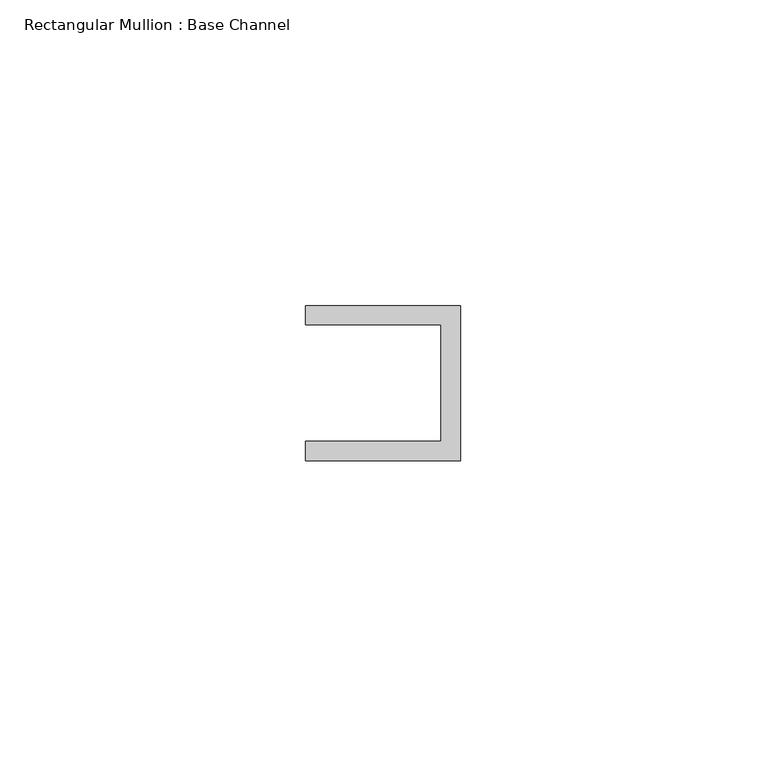
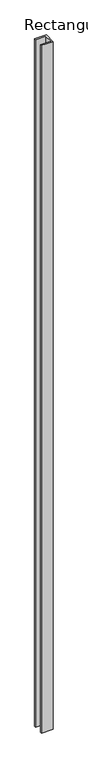
"""IFC4 building model written with IfcOpenShell, lengths in millimetres: member geometry, Rectangular Mullion : Base Channel."""

from ifc_helpers import new_model, si_unit, frame, origin, place, context, project, spatial, polyline, outline, extrude, source, transform, mapped, element, save


def rectangular_mullion_base_channel_9b0b3dad(model_context):
    return source(origin(), model_context, "Body", "SweptSolid", [
        extrude(outline(polyline([(0.0, 12.7), (0.0, -12.7), (-25.4, -12.7), (-25.4, -9.525), (-3.175, -9.525), (-3.175, 9.525), (-25.4, 9.525), (-25.4, 12.7), (0.0, 12.7)])), frame((0.0, 0.0, -1581.15), z_axis=(0.0, 0.0, 1.0), x_axis=(1.0, 0.0, 0.0)), (0.0, 0.0, 1.0), 1581.15),
    ])


if __name__ == "__main__":
    model = new_model("IFC4")
    model_context = context("Model", 3, world=origin())
    ifc_project = project(units=[si_unit("LENGTHUNIT", "METRE", prefix="MILLI")], contexts=[model_context])
    site = spatial("IfcSite", under=ifc_project)
    building = spatial("IfcBuilding", under=site)
    placement = place(None, origin())
    rectangular_mullion_base_channel_shape = rectangular_mullion_base_channel_9b0b3dad(model_context)
    element("IfcMember", 1, ObjectType="Rectangular Mullion : Base Channel", at=placement, inside=building, context=model_context, shape_type="MappedRepresentation", body=[
        mapped(rectangular_mullion_base_channel_shape, transform((0.0, 0.0, 0.0), x_axis=(1.0, 0.0, 0.0), y_axis=(0.0, 1.0, 0.0), z_axis=(0.0, 0.0, 1.0))),
    ])
    save(model, "model.ifc")

# Revit data of these elements
# Type "Rectangular Mullion : Base Channel"
#   built-in parameter 1007322 = 0.0833333 (stored number, unit not read)
#   built-in parameter 1007321 = 0.0416667 (stored number, unit not read)
#   built-in parameter 1007320 = -0.03125 (stored number, unit not read)
# Element 1 (IfcMember, "Rectangular Mullion : Base Channel")
#   Materials on its faces: "ALUM"
# Materials
#   "ALUM": class "Generic", colour RGB 157 157 157, transparency 0, Cost = 0
